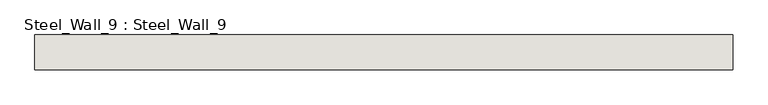
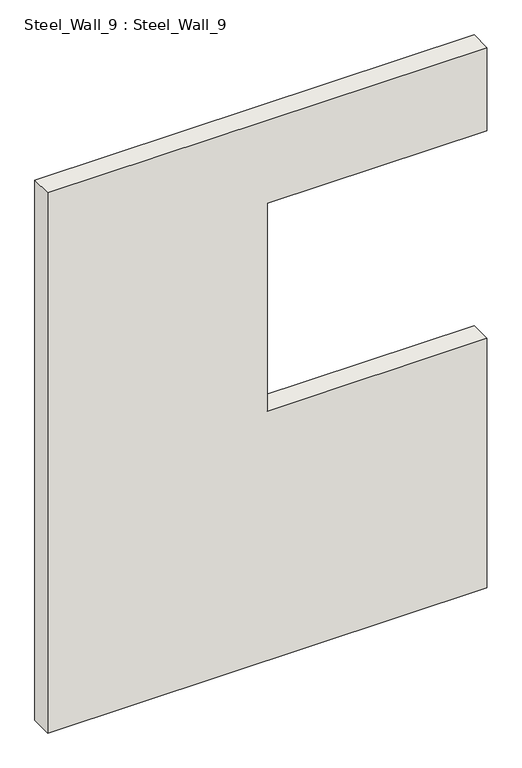
"""IFC4 building model written with IfcOpenShell, lengths in millimetres: wall geometry, Steel_Wall_9 : Steel_Wall_9."""

from ifc_helpers import new_model, si_unit, frame, origin, place, context, project, spatial, polyline, outline, extrude, source, transform, mapped, element, save


def steel_wall_9_steel_wall_9_7bb1e214(model_context):
    return source(origin(), model_context, "Body", "SweptSolid", [
        extrude(outline(polyline([(2850.0, 6075.0), (2850.0, 4075.0), (250.0, 4075.0), (250.0, 6075.0), (1450.0, 6075.0), (1450.0, 5075.0), (2450.0, 5075.0), (2450.0, 6075.0), (2850.0, 6075.0)])), frame((0.0, 12105.0, 0.0), z_axis=(0.0, 1.0, 0.0), x_axis=(0.0, 0.0, 1.0)), (0.0, 0.0, 1.0), 100.0),
    ])


if __name__ == "__main__":
    model = new_model("IFC4")
    model_context = context("Model", 3, world=origin())
    ifc_project = project(units=[si_unit("LENGTHUNIT", "METRE", prefix="MILLI")], contexts=[model_context])
    site = spatial("IfcSite", under=ifc_project)
    building = spatial("IfcBuilding", under=site)
    placement = place(None, origin())
    steel_wall_9_steel_wall_9_shape = steel_wall_9_steel_wall_9_7bb1e214(model_context)
    element("IfcWall", 1, ObjectType="Steel_Wall_9 : Steel_Wall_9", at=placement, inside=building, context=model_context, shape_type="MappedRepresentation", body=[
        mapped(steel_wall_9_steel_wall_9_shape, transform((0.0, 0.0, 0.0), x_axis=(1.0, 0.0, 0.0), y_axis=(0.0, 1.0, 0.0), z_axis=(0.0, 0.0, 1.0))),
    ])
    save(model, "model.ifc")

# Revit data of these elements
# Type "Steel_Wall_9 : Steel_Wall_9"
#   NameOverride = "Steel_Wall_9"
# Element 1 (IfcWall, "Steel_Wall_9 : Steel_Wall_9")
#   Materials on its faces: "IfcSurfaceStyle #33"
# Materials
#   "IfcSurfaceStyle #33": class "Unassigned", colour RGB 214 214 214, transparency 0
